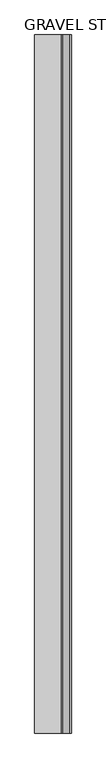
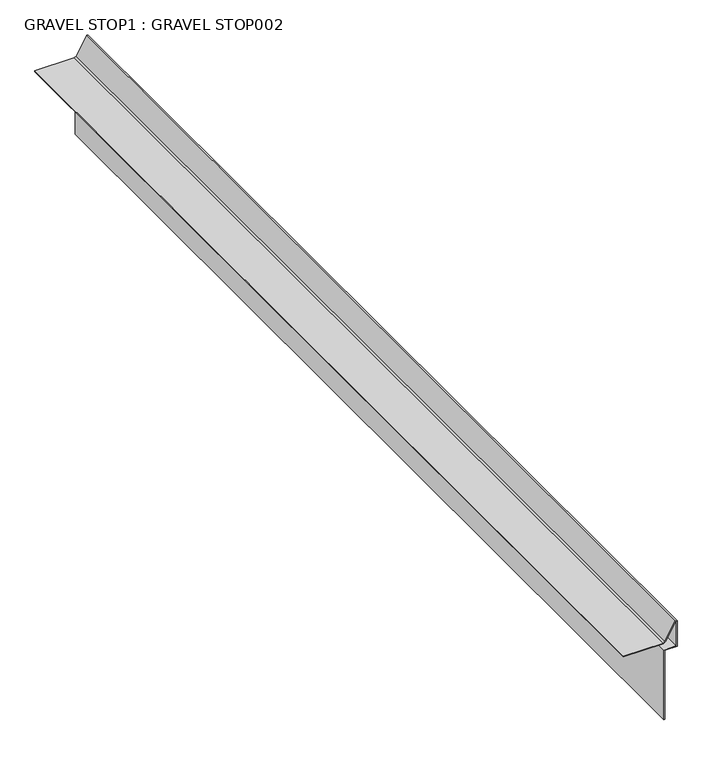
"""IFC4 building model written with IfcOpenShell, lengths in millimetres: proxy geometry, GRAVEL STOP1 : GRAVEL STOP002."""

from ifc_helpers import new_model, si_unit, frame, origin, place, context, project, spatial, polyline, outline, extrude, source, transform, mapped, element, save


def gravel_stop1_gravel_stop002_7041c615(model_context):
    return source(origin(), model_context, "Body", "SweptSolid", [
        extrude(outline(polyline([(40295.3431515, -4364.7039765), (40259.5408757, -4385.3744301), (40257.3744784, -4389.1267403), (40257.3744784, -4466.584647), (40255.9633674, -4466.584647), (40255.9633674, -4388.7486343), (40258.5078708, -4384.3414252), (40293.699878, -4364.0233103), (40293.447969, -4363.0831732), (40242.3744784, -4363.0831732), (40242.3744784, -4387.4229108), (40097.9858473, -4387.4229108), (40097.9858473, -4386.0117998), (40240.9633674, -4386.0117998), (40240.9633674, -4361.6720622), (40294.5307525, -4361.6720622), (40295.3431515, -4364.7039765)])), frame((0.0, -1052.8906573, 0.0), z_axis=(0.0, 1.0, 0.0), x_axis=(0.0, 0.0, 1.0)), (0.0, 0.0, 1.0), 2000.25),
    ])


if __name__ == "__main__":
    model = new_model("IFC4")
    model_context = context("Model", 3, world=origin())
    ifc_project = project(units=[si_unit("LENGTHUNIT", "METRE", prefix="MILLI")], contexts=[model_context])
    site = spatial("IfcSite", under=ifc_project)
    building = spatial("IfcBuilding", under=site)
    placement = place(None, origin())
    gravel_stop1_gravel_stop002_shape = gravel_stop1_gravel_stop002_7041c615(model_context)
    element("IfcBuildingElementProxy", 1, Name="GRAVEL STOP1 : GRAVEL STOP002", ObjectType="GRAVEL STOP1 : GRAVEL STOP002", at=placement, inside=building, context=model_context, shape_type="MappedRepresentation", body=[
        mapped(gravel_stop1_gravel_stop002_shape, transform((0.0, 0.0, 0.0), x_axis=(1.0, 0.0, 0.0), y_axis=(0.0, 1.0, 0.0), z_axis=(0.0, 0.0, 1.0))),
    ])
    save(model, "model.ifc")

# Revit data of these elements
# Type "GRAVEL STOP1 : GRAVEL STOP002"
#   NameOverride = "GRAVEL STOP002"
# Element 1 (IfcBuildingElementProxy, "GRAVEL STOP1 : GRAVEL STOP002")
#   Materials on its faces: "GRAVEL STOP REQUIRED WITH GRAVEL SURFACE SYSTEMS"
# Materials
#   "GRAVEL STOP REQUIRED WITH GRAVEL SURFACE SYSTEMS": class "Unassigned", colour RGB 170 170 127, transparency 0, Cost = 0
